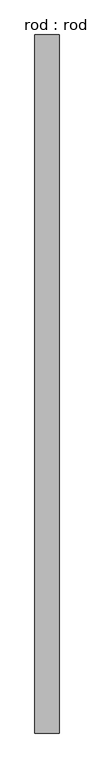
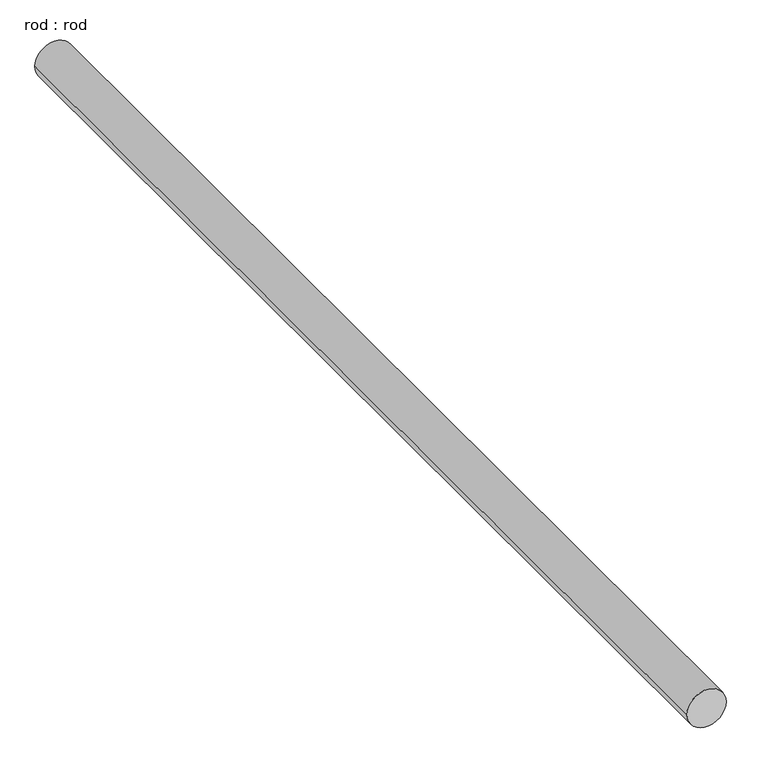
"""IFC4 building model written with IfcOpenShell, lengths in millimetres: proxy geometry, rod : rod."""

from ifc_helpers import new_model, si_unit, point, frame, frame_2d, origin, place, context, project, spatial, circle_curve, trimmed, segment, composite_curve, outline, extrude, source, transform, mapped, element, save


def rod_rod_23e402c4(model_context):
    return source(origin(), model_context, "Body", "SweptSolid", [
        extrude(outline(composite_curve([segment(trimmed(circle_curve(frame_2d((0.0108462, 0.0)), 200.0), [point((0.0108462, 200.0))], [point((0.0108462, -200.0))], False, "CARTESIAN"), True, "CONTINUOUS"), segment(trimmed(circle_curve(frame_2d((0.0108462, 0.0)), 200.0), [point((0.0108462, -200.0))], [point((0.0108462, 200.0))], False, "CARTESIAN"), True, "CONTINUOUS")], self_intersect=False)), frame((0.0, -1692.9856704, 0.0), z_axis=(0.0, 1.0, 0.0), x_axis=(0.0, 0.0, 1.0)), (0.0, 0.0, 1.0), 11571.4285714),
    ])


if __name__ == "__main__":
    model = new_model("IFC4")
    model_context = context("Model", 3, world=origin())
    ifc_project = project(units=[si_unit("LENGTHUNIT", "METRE", prefix="MILLI")], contexts=[model_context])
    site = spatial("IfcSite", under=ifc_project)
    building = spatial("IfcBuilding", under=site)
    placement = place(None, origin())
    rod_rod_shape = rod_rod_23e402c4(model_context)
    element("IfcBuildingElementProxy", 1, Name="rod : rod", ObjectType="rod : rod", at=placement, inside=building, context=model_context, shape_type="MappedRepresentation", body=[
        mapped(rod_rod_shape, transform((0.0, 0.0, 0.0), x_axis=(1.0, 0.0, 0.0), y_axis=(0.0, 1.0, 0.0), z_axis=(0.0, 0.0, 1.0))),
    ])
    save(model, "model.ifc")

# Revit data of these elements
# Type "rod : rod"
#   Default Elevation = 0
